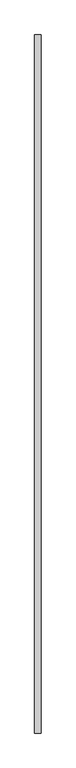
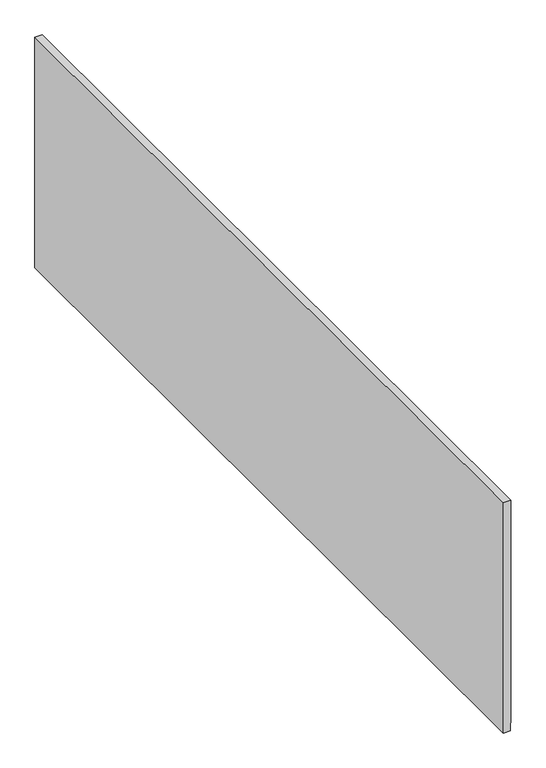
"""IFC4 building model written with IfcOpenShell, lengths in millimetres: proxy geometry, Gypsum027 11457 : Gypsum027 11457."""

from ifc_helpers import new_model, si_unit, frame, origin, place, context, project, spatial, polyline, outline, extrude, source, transform, mapped, element, save


def generic_models_bfbcf28b(model_context):
    return source(origin(), model_context, "Body", "SweptSolid", [
        extrude(outline(polyline([(35656.0216362, -8269.6582011), (35055.7176364, -8269.6582011), (35055.7176364, -8253.1630283), (35076.8706722, -8253.1630283), (35076.8706722, -8251.8779965), (35656.0216362, -8251.8779965), (35656.0216362, -8269.6582011)])), frame((0.0, 4540.4513986, 0.0), z_axis=(0.0, 1.0, 0.0), x_axis=(0.0, 0.0, 1.0)), (0.0, 0.0, 1.0), 2000.0),
    ])


if __name__ == "__main__":
    model = new_model("IFC4")
    model_context = context("Model", 3, world=origin())
    ifc_project = project(units=[si_unit("LENGTHUNIT", "METRE", prefix="MILLI")], contexts=[model_context])
    site = spatial("IfcSite", under=ifc_project)
    building = spatial("IfcBuilding", under=site)
    placement = place(None, origin())
    generic_models_shape = generic_models_bfbcf28b(model_context)
    element("IfcBuildingElementProxy", 1, Name="Gypsum027 11457 : Gypsum027 11457", ObjectType="Gypsum027 11457 : Gypsum027 11457", at=placement, inside=building, context=model_context, shape_type="MappedRepresentation", body=[
        mapped(generic_models_shape, transform((0.0, 0.0, 0.0), x_axis=(1.0, 0.0, 0.0), y_axis=(0.0, 1.0, 0.0), z_axis=(0.0, 0.0, 1.0))),
    ])
    save(model, "model.ifc")

# Revit data of these elements
# Type "Gypsum027 11457 : Gypsum027 11457"
#   NameOverride = "Gypsum027"
# Element 1 (IfcBuildingElementProxy, "Gypsum027 11457 : Gypsum027 11457")
#   Materials on its faces: "5/8\" GYPSUM BOARD"
# Materials
#   "5/8\" GYPSUM BOARD": class "Unassigned", colour RGB 255 255 255, transparency 0, Cost = 0
